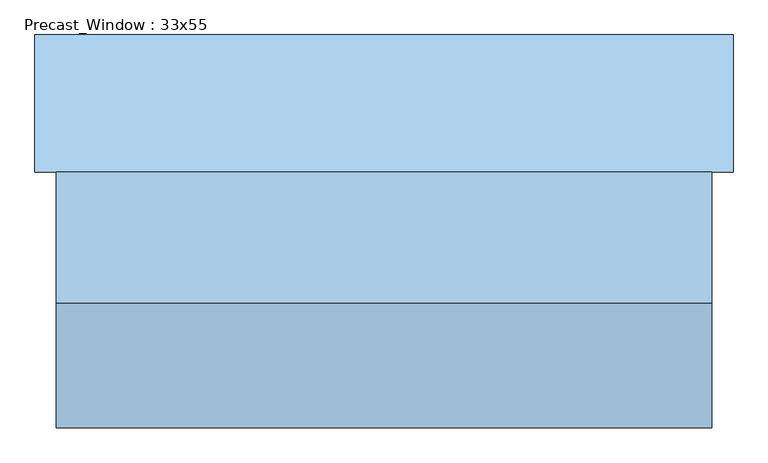
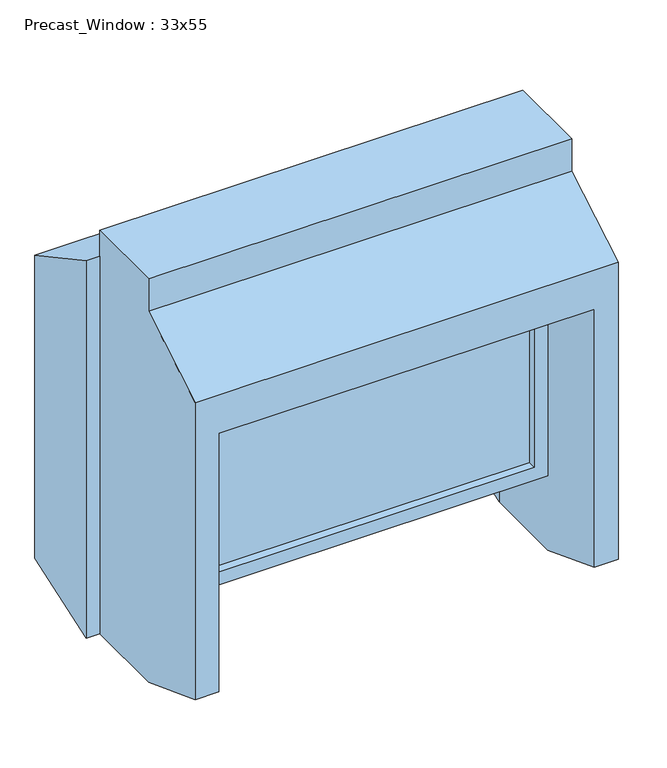
"""IFC4 building model written with IfcOpenShell, lengths in millimetres: window geometry, Precast_Window : 33x55."""

from ifc_helpers import new_model, si_unit, frame, origin, place, context, project, spatial, polyline, outline, extrude, faceted_brep, source, transform, mapped, element, save


def precast_window_33x55_2f7ce484(model_context):
    return source(origin(), model_context, "Body", "SolidModel", [
        extrude(outline(polyline([(647.7, -106.3625), (647.7, -125.4125), (-647.7, -125.4125), (-647.7, -106.3625), (647.7, -106.3625)])), frame((0.0, 0.0, 1066.8), z_axis=(0.0, 0.0, 1.0), x_axis=(1.0, 0.0, 0.0)), (0.0, 0.0, 1.0), 736.6),
        extrude(outline(polyline([(1854.2, -698.5), (1016.0, -698.5), (1016.0, 698.5), (1854.2, 698.5), (1854.2, -698.5)]), holes=[polyline([(1803.4, -647.7), (1803.4, 647.7), (1066.8, 647.7), (1066.8, -647.7), (1803.4, -647.7)])]), frame((0.0, -157.1625, 0.0), z_axis=(0.0, 1.0, 0.0), x_axis=(0.0, 0.0, 1.0)), (0.0, 0.0, 1.0), 101.6),
        faceted_brep([(838.2, 157.1625, 723.9), (838.2, 487.3625, 838.2), (838.2, 487.3625, 2032.0), (838.2, 157.1625, 2209.8), (698.5, 157.1625, 1854.2), (698.5, 157.1625, 723.9), (-838.2, 157.1625, 2209.8), (-838.2, 157.1625, 723.9), (-698.5, 157.1625, 723.9), (-698.5, 157.1625, 1854.2), (698.5, 487.3625, 838.2), (698.5, 487.3625, 1854.2), (-698.5, 487.3625, 1854.2), (-698.5, 487.3625, 838.2), (-838.2, 487.3625, 838.2), (-838.2, 487.3625, 2032.0)], [[[0, 1, 2, 3]], [[4, 5, 0, 3, 6, 7, 8, 9]], [[1, 0, 5, 10]], [[10, 11, 12, 13, 14, 15, 2, 1]], [[11, 10, 5, 4]], [[13, 8, 7, 14]], [[9, 8, 13, 12]], [[11, 4, 9, 12]], [[7, 6, 15, 14]], [[3, 2, 15, 6]]]),
        faceted_brep([(787.4, -457.2, 838.2), (787.4, -157.1625, 723.9), (787.4, 157.1625, 723.9), (787.4, 157.1625, 2311.4), (787.4, -157.1625, 2311.4), (787.4, -157.1625, 2184.4), (787.4, -457.2, 2006.6), (698.5, 157.1625, 723.9), (698.5, 157.1625, 1854.2), (-698.5, 157.1625, 1854.2), (-698.5, 157.1625, 723.9), (-787.4, 157.1625, 723.9), (-787.4, 157.1625, 2311.4), (698.5, -457.2, 1854.2), (698.5, -457.2, 838.2), (-787.4, -457.2, 2006.6), (-787.4, -457.2, 838.2), (-698.5, -457.2, 838.2), (-698.5, -457.2, 1854.2), (698.5, -157.1625, 723.9), (-787.4, -157.1625, 2184.4), (-787.4, -157.1625, 2311.4), (-787.4, -157.1625, 723.9), (-698.5, -157.1625, 723.9)], [[[0, 1, 2, 3, 4, 5, 6]], [[7, 8, 9, 10, 11, 12, 3, 2]], [[13, 14, 0, 6, 15, 16, 17, 18]], [[8, 7, 19, 14, 13]], [[16, 15, 20, 21, 12, 11, 22]], [[18, 17, 23, 10, 9]], [[8, 13, 18, 9]], [[4, 3, 12, 21]], [[5, 4, 21, 20]], [[6, 5, 20, 15]], [[1, 0, 14, 19]], [[2, 1, 19, 7]], [[10, 23, 22, 11]], [[23, 17, 16, 22]]]),
    ])


if __name__ == "__main__":
    model = new_model("IFC4")
    model_context = context("Model", 3, world=origin())
    ifc_project = project(units=[si_unit("LENGTHUNIT", "METRE", prefix="MILLI")], contexts=[model_context])
    site = spatial("IfcSite", under=ifc_project)
    building = spatial("IfcBuilding", under=site)
    placement = place(None, origin())
    precast_window_33x55_shape = precast_window_33x55_2f7ce484(model_context)
    element("IfcWindow", 1, ObjectType="Precast_Window : 33x55", at=placement, inside=building, context=model_context, shape_type="MappedRepresentation", body=[
        mapped(precast_window_33x55_shape, transform((0.0, 0.0, 0.0), x_axis=(1.0, 0.0, 0.0), y_axis=(0.0, 1.0, 0.0), z_axis=(0.0, 0.0, 1.0))),
    ])
    save(model, "model.ifc")

# Revit data of these elements
# Type "Precast_Window : 33x55"
#   Type Mark = "25"
#   Analytic Construction = "<None>"
#   Height = 2' - 9"
#   Frame Width = 0' - 2"
#   Default Sill Height = 4' - 0"
#   Width = 4' - 7"
#   Precast Material = Stucco - Plaster Cement - Taupe
#   Frame Material = Metal Trim
#   Wall Closure = (empty or 0)
# Element 1 (IfcWindow, "Precast_Window : 33x55")
#   Materials on its faces: "Stucco - Plaster Cement - Taupe", "Metal Trim", "Glass"
# Materials
#   "Stucco - Plaster Cement - Taupe": class "Generic", colour RGB 137 123 107, transparency 0, Description = "Gypsum Wall Board", Cost = 0
#   "Metal Trim": class "Wood", colour RGB 151 137 121, transparency 0, Cost = 0
#   "Glass": class "Glass", colour RGB 218 227 224, transparency 0.85, Description = "Soda Lime Glass", Cost = 0
